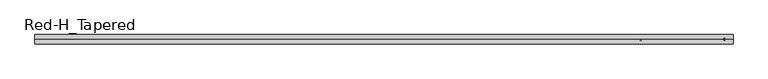
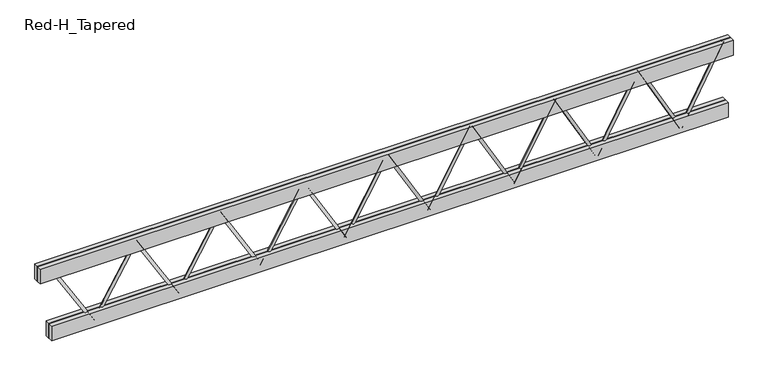
"""IFC4 building model written with IfcOpenShell, lengths in millimetres: beam geometry, Construction_Frames_RedBuilt_Openweb_Red-H_Tapered : Red-H_Tapered."""

from ifc_helpers import new_model, si_unit, point, frame, origin, origin_2d, place, context, project, spatial, polyline, circle_curve, trimmed, segment, composite_curve, outline, extrude, source, transform, mapped, element, save


def red_h_tapered_c050dafc(model_context):
    return source(origin(), model_context, "Body", "SweptSolid", [
        extrude(outline(composite_curve([segment(trimmed(circle_curve(origin_2d(), 12.7), [point((0.0, -12.7))], [point((0.0, 12.7))], False, "CARTESIAN"), True, "CONTINUOUS"), segment(trimmed(circle_curve(origin_2d(), 12.7), [point((0.0, 12.7))], [point((0.0, -12.7))], False, "CARTESIAN"), True, "CONTINUOUS")], self_intersect=False)), frame((2613.6132728, 0.0, -417.8101562), z_axis=(0.47816167222020944, 0.0, 0.8782718344678788), x_axis=(0.0, 1.0, 0.0)), (0.0, 0.0, 1.0), 780.8516374),
        extrude(outline(composite_curve([segment(trimmed(circle_curve(origin_2d(), 12.7), [point((0.0, 12.7000001))], [point((0.0, -12.6999999))], False, "CARTESIAN"), True, "CONTINUOUS"), segment(trimmed(circle_curve(origin_2d(), 12.7), [point((0.0, -12.6999999))], [point((0.0, 12.7000001))], False, "CARTESIAN"), True, "CONTINUOUS")], self_intersect=False)), frame((2613.6132728, 0.0, -417.8101562), z_axis=(-0.4828970273635993, 0.0, 0.875677144250893), x_axis=(0.0, 1.0, 0.0)), (0.0, 0.0, 1.0), 773.194498),
        extrude(outline(composite_curve([segment(trimmed(circle_curve(origin_2d(), 12.7), [point((0.0, -12.7))], [point((0.0, 12.6999999))], False, "CARTESIAN"), True, "CONTINUOUS"), segment(trimmed(circle_curve(origin_2d(), 12.7), [point((0.0, 12.6999999))], [point((0.0, -12.7))], False, "CARTESIAN"), True, "CONTINUOUS")], self_intersect=False)), frame((1866.8666234, 0.0, -417.8101562), z_axis=(0.48289702736359963, 0.0, 0.8756771442508928), x_axis=(0.0, 1.0, 0.0)), (0.0, 0.0, 1.0), 773.194498),
        extrude(outline(composite_curve([segment(trimmed(circle_curve(origin_2d(), 12.7), [point((0.0, 12.7))], [point((0.0, -12.6999999))], False, "CARTESIAN"), True, "CONTINUOUS"), segment(trimmed(circle_curve(origin_2d(), 12.7), [point((0.0, -12.6999999))], [point((0.0, 12.7))], False, "CARTESIAN"), True, "CONTINUOUS")], self_intersect=False)), frame((1866.8666234, 0.0, -417.8101562), z_axis=(-0.4877124623909616, 0.0, 0.8730043264661091), x_axis=(0.0, 1.0, 0.0)), (0.0, 0.0, 1.0), 765.5603526),
        extrude(outline(composite_curve([segment(trimmed(circle_curve(origin_2d(), 12.7), [point((0.0, -12.7000001))], [point((0.0, 12.6999999))], False, "CARTESIAN"), True, "CONTINUOUS"), segment(trimmed(circle_curve(origin_2d(), 12.7), [point((0.0, 12.6999999))], [point((0.0, -12.7000001))], False, "CARTESIAN"), True, "CONTINUOUS")], self_intersect=False)), frame((1120.119974, 0.0, -417.8101562), z_axis=(0.4877124623909606, 0.0, 0.8730043264661097), x_axis=(0.0, 1.0, 0.0)), (0.0, 0.0, 1.0), 765.5603526),
        extrude(outline(composite_curve([segment(trimmed(circle_curve(origin_2d(), 12.7), [point((0.0, 12.7))], [point((0.0, -12.7000001))], False, "CARTESIAN"), True, "CONTINUOUS"), segment(trimmed(circle_curve(origin_2d(), 12.7), [point((0.0, -12.7000001))], [point((0.0, 12.7))], False, "CARTESIAN"), True, "CONTINUOUS")], self_intersect=False)), frame((1120.119974, 0.0, -417.8101562), z_axis=(-0.49260950720350616, 0.0, 0.8702504659077861), x_axis=(0.0, 1.0, 0.0)), (0.0, 0.0, 1.0), 757.9498959),
        extrude(outline(composite_curve([segment(trimmed(circle_curve(origin_2d(), 12.7), [point((0.0, -12.7))], [point((0.0, 12.7))], False, "CARTESIAN"), True, "CONTINUOUS"), segment(trimmed(circle_curve(origin_2d(), 12.7), [point((0.0, 12.7))], [point((0.0, -12.7))], False, "CARTESIAN"), True, "CONTINUOUS")], self_intersect=False)), frame((373.3733247, 0.0, -417.8101562), z_axis=(0.4926095072035067, 0.0, 0.870250465907786), x_axis=(0.0, 1.0, 0.0)), (0.0, 0.0, 1.0), 757.9498959),
        extrude(outline(composite_curve([segment(trimmed(circle_curve(origin_2d(), 12.7), [point((0.0, 12.7000001))], [point((0.0, -12.6999999))], False, "CARTESIAN"), True, "CONTINUOUS"), segment(trimmed(circle_curve(origin_2d(), 12.7), [point((0.0, -12.6999999))], [point((0.0, 12.7000001))], False, "CARTESIAN"), True, "CONTINUOUS")], self_intersect=False)), frame((373.3733247, 0.0, -417.8101562), z_axis=(-0.49758970318604673, 0.0, 0.8674125242831244), x_axis=(0.0, 1.0, 0.0)), (0.0, 0.0, 1.0), 750.3638485),
        extrude(outline(composite_curve([segment(trimmed(circle_curve(origin_2d(), 12.7), [point((0.0, 12.6999999))], [point((0.0, -12.7000001))], False, "CARTESIAN"), True, "CONTINUOUS"), segment(trimmed(circle_curve(origin_2d(), 12.7), [point((0.0, -12.7000001))], [point((0.0, 12.6999999))], False, "CARTESIAN"), True, "CONTINUOUS")], self_intersect=False)), frame((-373.3733247, 0.0, -417.8101562), z_axis=(0.4975897031860168, 0.0, 0.8674125242831416), x_axis=(0.0, 1.0, 0.0)), (0.0, 0.0, 1.0), 750.3638485),
        extrude(outline(composite_curve([segment(trimmed(circle_curve(origin_2d(), 12.7), [point((0.0, -12.7))], [point((0.0, 12.7))], False, "CARTESIAN"), True, "CONTINUOUS"), segment(trimmed(circle_curve(origin_2d(), 12.7), [point((0.0, 12.7))], [point((0.0, -12.7))], False, "CARTESIAN"), True, "CONTINUOUS")], self_intersect=False)), frame((-373.3733247, 0.0, -417.8101562), z_axis=(-0.5026546008969804, 0.0, 0.8644873348968725), x_axis=(0.0, 1.0, 0.0)), (0.0, 0.0, 1.0), 742.8029586),
        extrude(outline(composite_curve([segment(trimmed(circle_curve(origin_2d(), 12.7), [point((0.0, 12.7))], [point((0.0, -12.7))], False, "CARTESIAN"), True, "CONTINUOUS"), segment(trimmed(circle_curve(origin_2d(), 12.7), [point((0.0, -12.7))], [point((0.0, 12.7))], False, "CARTESIAN"), True, "CONTINUOUS")], self_intersect=False)), frame((-1120.119974, 0.0, -417.8101562), z_axis=(0.5026546008969787, 0.0, 0.8644873348968735), x_axis=(0.0, 1.0, 0.0)), (0.0, 0.0, 1.0), 742.8029586),
        extrude(outline(composite_curve([segment(trimmed(circle_curve(origin_2d(), 12.7), [point((0.0, -12.6999999))], [point((0.0, 12.7000001))], False, "CARTESIAN"), True, "CONTINUOUS"), segment(trimmed(circle_curve(origin_2d(), 12.7), [point((0.0, 12.7000001))], [point((0.0, -12.6999999))], False, "CARTESIAN"), True, "CONTINUOUS")], self_intersect=False)), frame((-1120.119974, 0.0, -417.8101562), z_axis=(-0.5078057574570192, 0.0, 0.8614715971484511), x_axis=(0.0, 1.0, 0.0)), (0.0, 0.0, 1.0), 735.268002),
        extrude(outline(composite_curve([segment(trimmed(circle_curve(origin_2d(), 12.7), [point((0.0, 12.7))], [point((0.0, -12.7000001))], False, "CARTESIAN"), True, "CONTINUOUS"), segment(trimmed(circle_curve(origin_2d(), 12.7), [point((0.0, -12.7000001))], [point((0.0, 12.7))], False, "CARTESIAN"), True, "CONTINUOUS")], self_intersect=False)), frame((-1866.8666234, 0.0, -417.8101562), z_axis=(0.5078057574570315, 0.0, 0.8614715971484438), x_axis=(0.0, 1.0, 0.0)), (0.0, 0.0, 1.0), 735.268002),
        extrude(outline(composite_curve([segment(trimmed(circle_curve(origin_2d(), 12.7), [point((0.0, -12.7))], [point((0.0, 12.7000001))], False, "CARTESIAN"), True, "CONTINUOUS"), segment(trimmed(circle_curve(origin_2d(), 12.7), [point((0.0, 12.7000001))], [point((0.0, -12.7))], False, "CARTESIAN"), True, "CONTINUOUS")], self_intersect=False)), frame((-1866.8666234, 0.0, -417.8101562), z_axis=(-0.5130447336074959, 0.0, 0.8583618708433022), x_axis=(0.0, 1.0, 0.0)), (0.0, 0.0, 1.0), 727.7597843),
        extrude(outline(composite_curve([segment(trimmed(circle_curve(origin_2d(), 12.7), [point((0.0, 12.6999999))], [point((0.0, -12.7000001))], False, "CARTESIAN"), True, "CONTINUOUS"), segment(trimmed(circle_curve(origin_2d(), 12.7), [point((0.0, -12.7000001))], [point((0.0, 12.6999999))], False, "CARTESIAN"), True, "CONTINUOUS")], self_intersect=False)), frame((-2613.6132728, 0.0, -417.8101562), z_axis=(0.5130447336074847, 0.0, 0.8583618708433088), x_axis=(0.0, 1.0, 0.0)), (0.0, 0.0, 1.0), 727.7597843),
        extrude(outline(composite_curve([segment(trimmed(circle_curve(origin_2d(), 12.7), [point((0.0, -12.7))], [point((0.0, 12.7))], False, "CARTESIAN"), True, "CONTINUOUS"), segment(trimmed(circle_curve(origin_2d(), 12.7), [point((0.0, 12.7))], [point((0.0, -12.7))], False, "CARTESIAN"), True, "CONTINUOUS")], self_intersect=False)), frame((-2613.6132728, 0.0, -417.8101562), z_axis=(-0.5183730904077388, 0.0, 0.8551545703211381), x_axis=(0.0, 1.0, 0.0)), (0.0, 0.0, 1.0), 720.2791418),
        extrude(outline(polyline([(-3012.3865974, 41.275), (3012.3865974, 41.275), (3012.3865974, 3.175), (-3012.3865974, 3.175), (-3012.3865974, 41.275)])), frame((0.0, 0.0, -436.8601562), z_axis=(0.0, 0.0, 1.0), x_axis=(1.0, 0.0, 0.0)), (0.0, 0.0, 1.0), 139.7),
        extrude(outline(polyline([(-3012.3865974, -3.175), (3012.3865974, -3.175), (3012.3865974, -41.275), (-3012.3865974, -41.275), (-3012.3865974, -3.175)])), frame((0.0, 0.0, -436.8601562), z_axis=(0.0, 0.0, 1.0), x_axis=(1.0, 0.0, 0.0)), (0.0, 0.0, 1.0), 139.7),
        extrude(outline(polyline([(-3113.9865974, 41.275), (3057.6900998, 41.275), (3057.6900998, 3.175), (-3113.9865974, 3.175), (-3113.9865974, 41.275)])), frame((0.0, 0.0, 134.6398438), z_axis=(0.0, 0.0, 1.0), x_axis=(1.0, 0.0, 0.0)), (0.0, 0.0, 1.0), 139.7),
        extrude(outline(polyline([(-3113.9865974, -3.175), (3057.6900998, -3.175), (3057.6900998, -41.275), (-3113.9865974, -41.275), (-3113.9865974, -3.175)])), frame((0.0, 0.0, 134.6398438), z_axis=(0.0, 0.0, 1.0), x_axis=(1.0, 0.0, 0.0)), (0.0, 0.0, 1.0), 139.7),
    ])


if __name__ == "__main__":
    model = new_model("IFC4")
    model_context = context("Model", 3, world=origin())
    ifc_project = project(units=[si_unit("LENGTHUNIT", "METRE", prefix="MILLI")], contexts=[model_context])
    site = spatial("IfcSite", under=ifc_project)
    building = spatial("IfcBuilding", under=site)
    placement = place(None, origin())
    red_h_tapered_shape = red_h_tapered_c050dafc(model_context)
    element("IfcBeam", 1, ObjectType="Construction_Frames_RedBuilt_Openweb_Red-H_Tapered : Red-H_Tapered", at=placement, inside=building, context=model_context, shape_type="MappedRepresentation", body=[
        mapped(red_h_tapered_shape, transform((0.0, 0.0, 0.0), x_axis=(1.0, 0.0, 0.0), y_axis=(0.0, 1.0, 0.0), z_axis=(0.0, 0.0, 1.0))),
    ])
    save(model, "model.ifc")

# Revit data of these elements
# Type "Construction_Frames_RedBuilt_Openweb_Red-H_Tapered : Red-H_Tapered"
#   Youtube clip = ""
#   Weight Net (Kg) = "0"
#   Webs = "Up to 2\" diameter tubular steel"
#   Uniformat II Description = ""
#   Uniformat II Code = ""
#   Uniclass 2015 Name = "Softwood trusses"
#   Uniclass 2015 Code = "Pr_20_85_90_81"
#   Uniclass 2.0 Description = "Structural Framing Systems"
#   Uniclass 2.0 Code = "SS-15-10-75"
#   Uniclass 1.4 Description = "Trusses"
#   Uniclass 1.4 Code = "L3523"
#   UNSPSC Code = "30103606"
#   Technical description = "http://www.redbuilt.com/reference/literature-and-other-resources"
#   Region South America = "None"
#   Region Oceania = "None"
#   Region North America = "US"
#   Region Middle East = "None"
#   Region Europe = "None"
#   Region Asia = "None"
#   Region Antarctica = "None"
#   Region Africa = "None"
#   QR code = "http://bimobject.com/redbuilt/product/redbuilt-0003"
#   Product url = "http://www.redbuilt.com/products/default.aspx?id=2"
#   Product group = "Wood Trusses"
#   Product family = "Construction"
#   Product data url = "https://bimobject.com/redbuilt/product/redbuilt-0003"
#   Product certification = ""
#   Product SKU = "redbuilt-0003"
#   Product Page URL = "http://www.redbuilt.com/commercial-systems/red-m-red-h-open-web-trusses"
#   Product Guid = "2c5793f2-6ffb-4665-b825-cf90c048e711"
#   Product Documentation Link = "http://www.redbuilt.com/documents/OW_Guide_2017_07_LowRes_wLinks.pdf"
#   OmniClass Description = "Wood Trusses"
#   OmniClass Code = "23-13 35 19 13 17"
#   NBS Reference Description = ""
#   NBS Reference Code = ""
#   Material secondary = "Steel"
#   Material main = "CHARRED WOOD"
#   Masterformat 2014 Description = "Metal-Web Wood Joists"
#   Masterformat 2014 Code = "06 17 36"
#   Manufacturer name = "RedBuilt"
#   Manufacturer country = "United States"
#   Installation instructions = "http://www.redbuilt.com/documents/Installation_Sheets_Open-Web.pdf"
#   IFC Classification = ""
#   EAN code = ""
#   Design country = "United States"
#   Product Information = "http://redbuilt.com/products/default.aspx?id=2"
#   Model = "Red-H-Tapered"
#   Manufacturer URL = "http://redbuilt.com/"
#   Manufacturer = "RedBuilt™"
#   Description = "Open Web Truss"
#   Date of publishing = "8/17/2010"
#   Contact us = "http://redbuilt.com/contact/"
#   Chords = "Double 1½\" x 5½\" MSR lumber"
#   COBIe Type Category = ""
#   Brand url = "http://www.redbuilt.com"
#   BIMobject main category code = "construction"
#   BIMobject main category = "Construction"
#   BIMobject category code = "construction-frames-trusses"
#   BIMobject category = "Frames & Trusses"
#   Web Radius = 0' - 0 1/2"
#   Web Layout Offset Start [instance default] = 0' - 5"
#   Web Layout Offset End [instance default] = 0' - 5"
#   Web Diameter = 0' - 1"
#   TotalLength [instance default] = 20' - 0"
#   Span Minimum = 4' - 0"
#   Span Maximum = 70' - 0"
#   Span Limit [instance default] = 20' - 0"
#   Nominal width = 0' - 0"
#   Nominal height = 0' - 0"
#   Inner Depth Top [instance default] = 0' - 2.76372"
#   Depth Start [instance default] = 6' - 0"
#   Top Chord Length [instance default] = 20' - 1.19701"
#   TC Extension Start Aux [instance default] = 0' - 0"
#   TC Extension End Aux [instance default] = 0' - 0"
#   T-B Chord Length Difference L [instance default] = 0' - 4"
#   T-B Chord Length Difference [instance default] = 0' - 4"
#   Height 2 [instance default] = 6' - 0"
#   Depth Minimum at Wall = 2' - 0"
#   Depth Maximum at Wall = 6' - 0"
#   Depth Lower End [instance default] = 2' - 0"
#   Depth Higher End [instance default] = 6' - 0"
#   Depth End [instance default] = 2' - 0"
#   Depth 2 [instance default] = 2' - 0"
#   Chord Width = 0' - 3 1/4"
#   Chord Thickness = 0' - 1 1/2"
#   Chord Depth = 0' - 5 1/2"
#   Offset Start [instance default] = 0' - 0"
#   TC Extension Start [instance default] = 0' - 0"
#   End Panel = 0' - 5"
#   Offset End [instance default] = 0' - 0"
#   TC Extension End [instance default] = 0' - 0"
#   Length [instance default] = 20' - 0"
#   Angle [instance default] = 5.71059°
#   Span Limit Warning [instance default] = no
#   Edition number = 1
#   Top Bearing Start [instance default] = yes
#   Top Bearing End [instance default] = yes
#   Bottom Bearing Start [instance default] = no
#   Bottom Bearing End [instance default] = no
#   8 Panels [instance default] = yes
#   16 Panels [instance default] = no
#   12 Panels [instance default] = no
#   Web Material = RedBuilt-Steel, Galvanized
#   Clip Material = RedBuilt-Steel, Galvanized
#   Chords Material = OPEN WEB TRUSSES - WOOD TOP/BOTTOM CHORD - TUBE STEEL WEBS
#   URL = ""
#   Assembly Code = ""
# Element 1 (IfcBeam, "Construction_Frames_RedBuilt_Openweb_Red-H_Tapered : Red-H_Tapered")
#   TotalLength = 20' - 5.1958"
#   Span Limit = 20' - 5.1958"
#   Inner Depth Top = 0' - 2 3/4"
#   Depth Start = 5' - 0"
#   Top Chord Length = 20' - 5.1958"
#   Height 2 = 5' - 0"
#   Depth Lower End = 2' - 4"
#   Depth Higher End = 5' - 0"
#   Depth End = 2' - 4"
#   Depth 2 = 0' - 0"
#   Angle = 0.00°
#   Materials on its faces: "RedBuilt-Steel, Galvanized", "OPEN WEB TRUSSES - WOOD TOP/BOTTOM CHORD - TUBE STEEL WEBS"
# Materials
#   "RedBuilt-Steel, Galvanized": class "Metal", colour RGB 164 172 176, transparency 0, Manufacturer = "RedBuilt. LLC", Comments = "Openweb Metal Web", URL = "http://www.redbuilt.com/", Description = "Galvanized steel", Cost = 0
#   "OPEN WEB TRUSSES - WOOD TOP/BOTTOM CHORD - TUBE STEEL WEBS": class "Wood", colour RGB 198 202 183, transparency 0, Description = "Generic wood", Cost = 0
